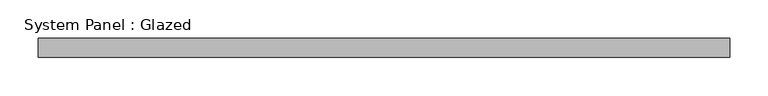
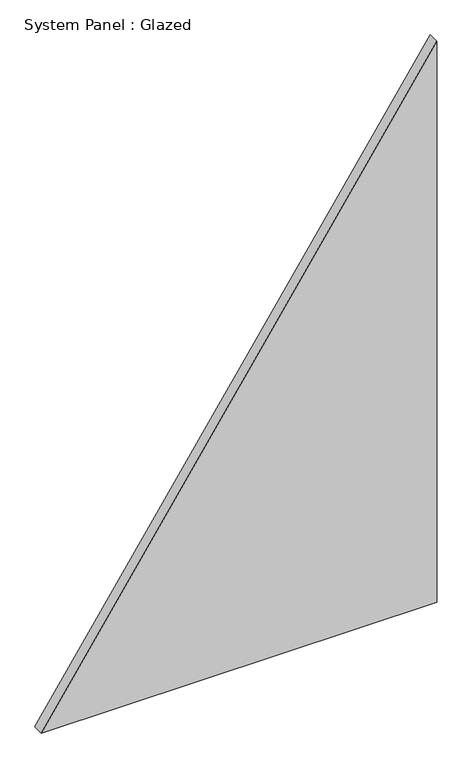
"""IFC4 building model written with IfcOpenShell, lengths in millimetres: plate geometry, System Panel : Glazed."""

from ifc_helpers import new_model, si_unit, frame, origin, place, context, project, spatial, polyline, outline, extrude, source, transform, mapped, element, save


def system_panel_glazed_3e781454(model_context):
    return source(origin(), model_context, "Body", "SweptSolid", [
        extrude(outline(polyline([(0.0, -453.2508456), (0.0, 453.2508456), (1359.5656239, 453.2508456), (0.0, -453.2508456)])), frame((0.0, 24.5, 0.0), z_axis=(0.0, 1.0, 0.0), x_axis=(0.0, 0.0, 1.0)), (0.0, 0.0, 1.0), 25.0),
    ])


if __name__ == "__main__":
    model = new_model("IFC4")
    model_context = context("Model", 3, world=origin())
    ifc_project = project(units=[si_unit("LENGTHUNIT", "METRE", prefix="MILLI")], contexts=[model_context])
    site = spatial("IfcSite", under=ifc_project)
    building = spatial("IfcBuilding", under=site)
    placement = place(None, origin())
    system_panel_glazed_shape = system_panel_glazed_3e781454(model_context)
    element("IfcPlate", 1, ObjectType="System Panel : Glazed", at=placement, inside=building, context=model_context, shape_type="MappedRepresentation", body=[
        mapped(system_panel_glazed_shape, transform((0.0, 0.0, 0.0), x_axis=(1.0, 0.0, 0.0), y_axis=(0.0, 1.0, 0.0), z_axis=(0.0, 0.0, 1.0))),
    ])
    save(model, "model.ifc")

# Revit data of these elements
# Type "System Panel : Glazed"
#   Keynote = "H11"
#   Construction Type Id = "GSP4R"
#   Analytic Construction = "1/8 in Pilkington single glazing"
#   Visual Light Transmittance = 0.9
#   Solar Heat Gain Coefficient = 0.86
#   Heat Transfer Coefficient (U) = 6.7069 W/(m²·K)
#   Define Thermal Properties by = 1
# Element 1 (IfcPlate, "System Panel : Glazed")
#   Materials on its faces: "Glass"
# Materials
#   "Glass": class "Glass", colour RGB 0 128 192, transparency 0.9, Description = "Soda Lime Glass", Cost = 0
